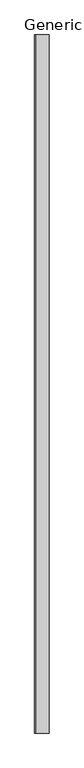
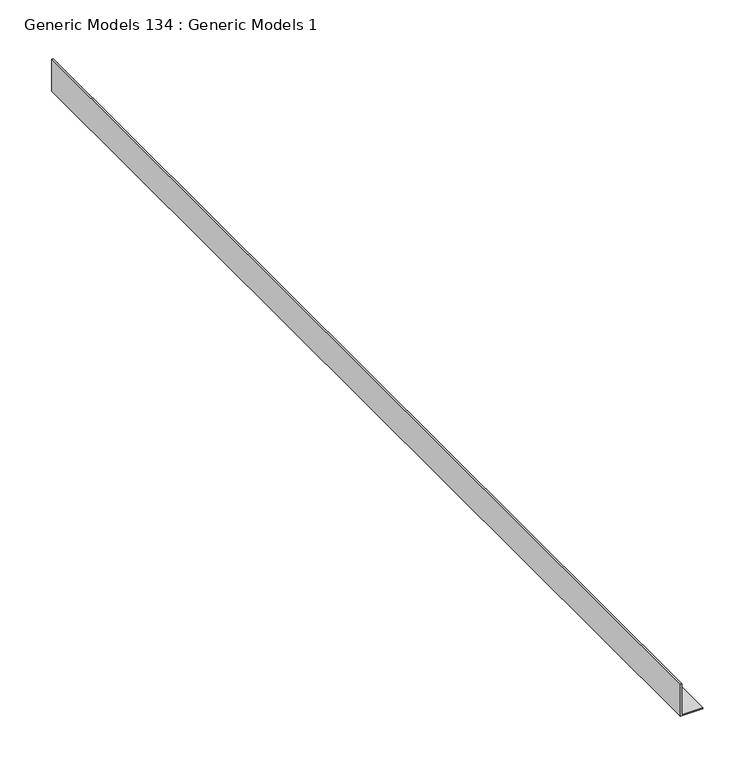
"""IFC4 building model written with IfcOpenShell, lengths in millimetres: proxy geometry, Generic Models 134 : Generic Models 1."""

from ifc_helpers import new_model, si_unit, frame, origin, place, context, project, spatial, polyline, outline, extrude, source, transform, mapped, element, save


def generic_models_134_generic_models_1_881594d0(model_context):
    return source(origin(), model_context, "Body", "SweptSolid", [
        extrude(outline(polyline([(2051.1444308, 46951.7485531), (2013.0444308, 46951.7485531), (2013.0444308, 46977.1485531), (2014.6319308, 46977.1485531), (2014.6319308, 46953.3360531), (2051.1444308, 46953.3360531), (2051.1444308, 46951.7485531)])), frame((0.0, 0.0, 0.0), z_axis=(0.0, 1.0, 0.0), x_axis=(0.0, 0.0, 1.0)), (0.0, 0.0, 1.0), 1219.2),
    ])


if __name__ == "__main__":
    model = new_model("IFC4")
    model_context = context("Model", 3, world=origin())
    ifc_project = project(units=[si_unit("LENGTHUNIT", "METRE", prefix="MILLI")], contexts=[model_context])
    site = spatial("IfcSite", under=ifc_project)
    building = spatial("IfcBuilding", under=site)
    placement = place(None, origin())
    generic_models_134_generic_models_1_shape = generic_models_134_generic_models_1_881594d0(model_context)
    element("IfcBuildingElementProxy", 1, Name="Generic Models 134 : Generic Models 1", ObjectType="Generic Models 134 : Generic Models 1", at=placement, inside=building, context=model_context, shape_type="MappedRepresentation", body=[
        mapped(generic_models_134_generic_models_1_shape, transform((0.0, 0.0, 0.0), x_axis=(1.0, 0.0, 0.0), y_axis=(0.0, 1.0, 0.0), z_axis=(0.0, 0.0, 1.0))),
    ])
    save(model, "model.ifc")

# Revit data of these elements
# Element 1 (IfcBuildingElementProxy, "Generic Models 134 : Generic Models 1")
#   Materials on its faces: "CEILING TRACK TO MATCH EXISTING"
# Materials
#   "CEILING TRACK TO MATCH EXISTING": class "Unassigned", colour RGB 210 209 208, transparency 0, Keynote = "M05121300.02", Cost = 0
